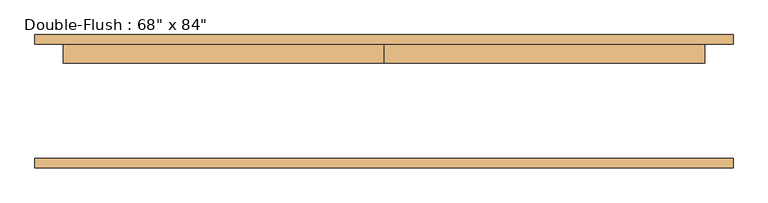
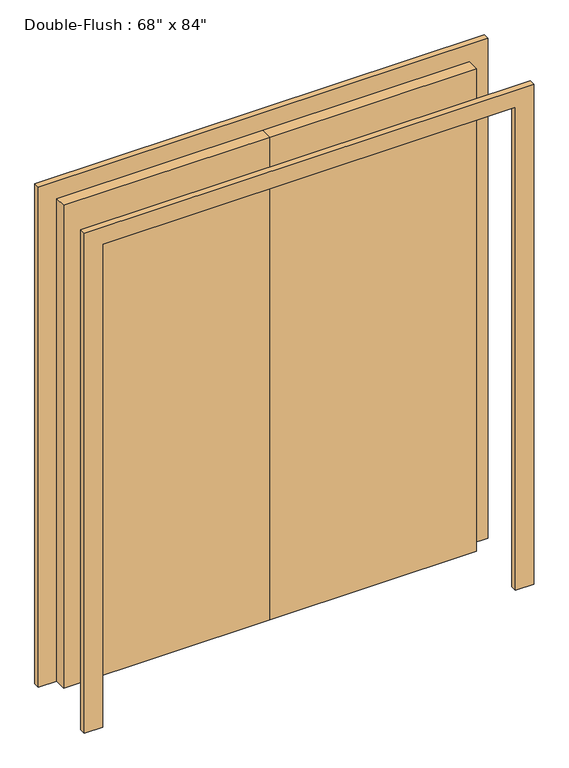
"""IFC4 building model written with IfcOpenShell, lengths in millimetres: door geometry."""

from ifc_helpers import new_model, si_unit, frame, origin, origin_with_axes, place, context, project, spatial, polyline, outline, extrude, source, transform, mapped, element, save


def door_bdee7c2d(model_context):
    return source(origin(), model_context, "Body", "SweptSolid", [
        extrude(outline(polyline([(0.0, 153.9875), (863.6, 153.9875), (863.6, 103.1875), (0.0, 103.1875), (0.0, 153.9875)])), origin_with_axes(), (0.0, 0.0, 1.0), 2133.6),
        extrude(outline(polyline([(-863.6, 153.9875), (0.0, 153.9875), (0.0, 103.1875), (-863.6, 103.1875), (-863.6, 153.9875)])), origin_with_axes(), (0.0, 0.0, 1.0), 2133.6),
        extrude(outline(polyline([(2133.6, -863.6), (2133.6, 863.6), (0.0, 863.6), (0.0, 939.8), (2209.8, 939.8), (2209.8, -939.8), (0.0, -939.8), (0.0, -863.6), (2133.6, -863.6)])), frame((0.0, -179.3875, 0.0), z_axis=(0.0, 1.0, 0.0), x_axis=(0.0, 0.0, 1.0)), (0.0, 0.0, 1.0), 25.4),
        extrude(outline(polyline([(2133.6, -863.6), (2133.6, 863.6), (0.0, 863.6), (0.0, 939.8), (2209.8, 939.8), (2209.8, -939.8), (0.0, -939.8), (0.0, -863.6), (2133.6, -863.6)])), frame((0.0, 153.9875, 0.0), z_axis=(0.0, 1.0, 0.0), x_axis=(0.0, 0.0, 1.0)), (0.0, 0.0, 1.0), 25.4),
    ])


if __name__ == "__main__":
    model = new_model("IFC4")
    model_context = context("Model", 3, world=origin())
    ifc_project = project(units=[si_unit("LENGTHUNIT", "METRE", prefix="MILLI")], contexts=[model_context])
    site = spatial("IfcSite", under=ifc_project)
    building = spatial("IfcBuilding", under=site)
    placement = place(None, origin())
    door_shape = door_bdee7c2d(model_context)
    element("IfcDoor", 1, ObjectType="Double-Flush : 68\" x 84\"", at=placement, inside=building, context=model_context, shape_type="MappedRepresentation", body=[
        mapped(door_shape, transform((0.0, 0.0, 0.0), x_axis=(1.0, 0.0, 0.0), y_axis=(0.0, 1.0, 0.0), z_axis=(0.0, 0.0, 1.0))),
    ])
    save(model, "model.ifc")

# Revit data of these elements
# Type "Double-Flush : 68\" x 84\""
#   Type Mark = "10"
#   Assembly Code = "C1020"
#   Thickness = 0' - 2"
#   Height = 7' - 0"
#   Trim Projection Ext = 0' - 1"
#   Trim Projection Int = 0' - 1"
#   Trim Width = 0' - 3"
#   Width = 5' - 8"
#   Function = 0
#   Door Material = Door - Panel
#   Frame Material = Door - Frame
#   Wall Closure = (empty or 0)
# Element 1 (IfcDoor, "Double-Flush : 68\" x 84\"")
#   Materials on its faces: "Door - Frame", "Door - Panel"
# Materials
#   "Door - Panel": class "Wood", colour RGB 210 159 95, transparency 0
#   "Door - Frame": class "Miscellaneous", colour RGB 118 70 51, transparency 0
